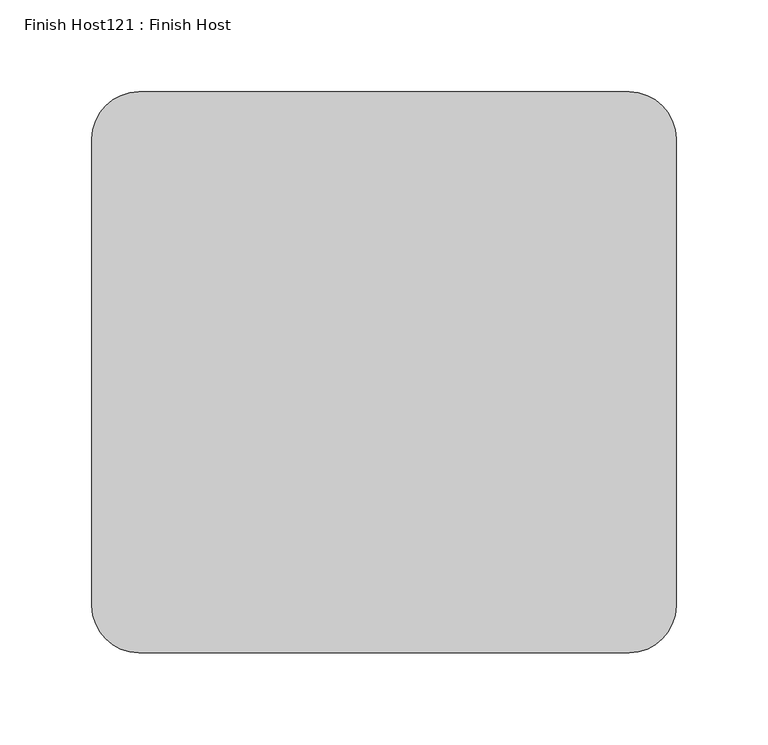
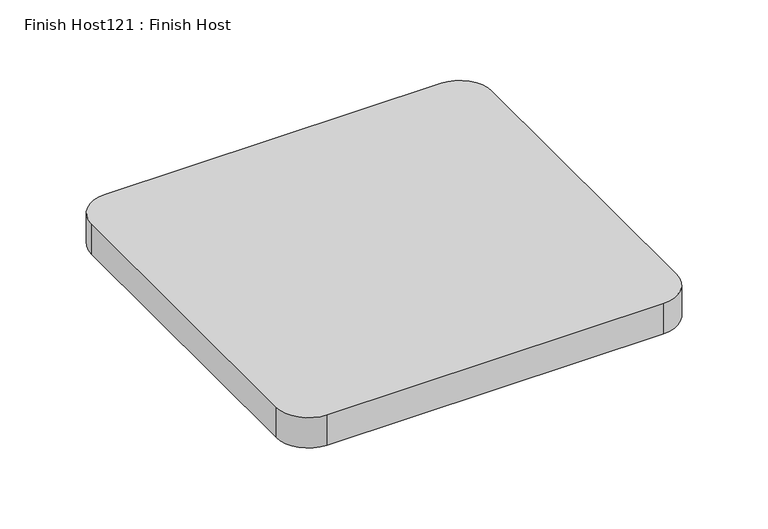
"""IFC4 building model written with IfcOpenShell, lengths in millimetres: proxy geometry, Finish Host121 : Finish Host."""

from ifc_helpers import new_model, si_unit, point, frame_2d, origin, origin_with_axes, place, context, project, spatial, polyline, circle_curve, trimmed, segment, composite_curve, outline, extrude, source, transform, mapped, element, save


def finish_host121_finish_host_94b01cf0(model_context):
    return source(origin(), model_context, "Body", "SweptSolid", [
        extrude(outline(composite_curve([segment(polyline([(-47.8842816, 3462.3960864), (-47.8842816, 3716.3960864)]), True, "CONTINUOUS"), segment(trimmed(circle_curve(frame_2d((-22.4842816, 3716.3960864)), 25.4), [point((-47.8842816, 3716.3960864))], [point((-22.4842816, 3741.7960864))], False, "CARTESIAN"), True, "CONTINUOUS"), segment(polyline([(-22.4842816, 3741.7960864), (244.2157184, 3741.7960864)]), True, "CONTINUOUS"), segment(trimmed(circle_curve(frame_2d((244.2157184, 3716.3960864)), 25.4), [point((244.2157184, 3741.7960864))], [point((269.6157184, 3716.3960864))], False, "CARTESIAN"), True, "CONTINUOUS"), segment(polyline([(269.6157184, 3716.3960864), (269.6157184, 3462.3960864)]), True, "CONTINUOUS"), segment(trimmed(circle_curve(frame_2d((244.2157184, 3462.3960864)), 25.4), [point((269.6157184, 3462.3960864))], [point((244.2157184, 3436.9960864))], False, "CARTESIAN"), True, "CONTINUOUS"), segment(polyline([(244.2157184, 3436.9960864), (-22.4842816, 3436.9960864)]), True, "CONTINUOUS"), segment(trimmed(circle_curve(frame_2d((-22.4842816, 3462.3960864)), 25.4), [point((-22.4842816, 3436.9960864))], [point((-47.8842816, 3462.3960864))], False, "CARTESIAN"), True, "CONTINUOUS")], self_intersect=False)), origin_with_axes(), (0.0, 0.0, 1.0), 25.4),
    ])


if __name__ == "__main__":
    model = new_model("IFC4")
    model_context = context("Model", 3, world=origin())
    ifc_project = project(units=[si_unit("LENGTHUNIT", "METRE", prefix="MILLI")], contexts=[model_context])
    site = spatial("IfcSite", under=ifc_project)
    building = spatial("IfcBuilding", under=site)
    placement = place(None, origin())
    finish_host121_finish_host_shape = finish_host121_finish_host_94b01cf0(model_context)
    element("IfcBuildingElementProxy", 1, Name="Finish Host121 : Finish Host", ObjectType="Finish Host121 : Finish Host", at=placement, inside=building, context=model_context, shape_type="MappedRepresentation", body=[
        mapped(finish_host121_finish_host_shape, transform((0.0, 0.0, 0.0), x_axis=(1.0, 0.0, 0.0), y_axis=(0.0, 1.0, 0.0), z_axis=(0.0, 0.0, 1.0))),
    ])
    save(model, "model.ifc")

# Revit data of these elements
# Type "Finish Host121 : Finish Host"
#   Countertop Material = Fabric - Teknion - R385 - Rationale - Mind's Eye
# Element 1 (IfcBuildingElementProxy, "Finish Host121 : Finish Host")
#   Materials on its faces: "Fabric - Teknion - R385 - Rationale - Mind's Eye"
# Materials
#   "Fabric - Teknion - R385 - Rationale - Mind's Eye": class "Fabric", colour RGB 40 41 40, transparency 0, Model = "R385", Manufacturer = "Teknion Studios", URL = "http://www.teknionstudio.com/", Description = "Mind's Eye Rationale", Cost = 0
